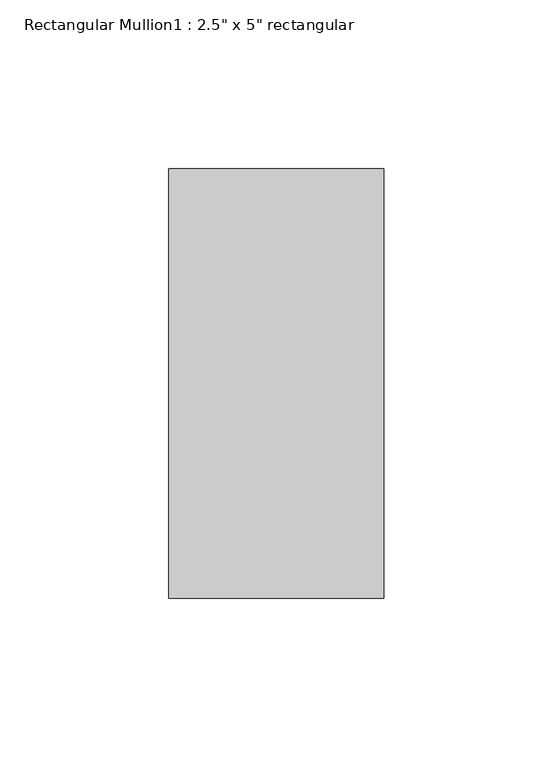
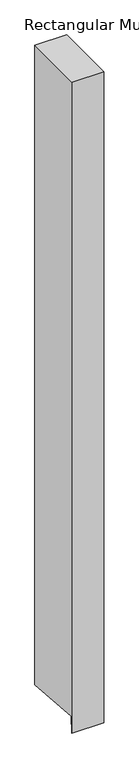
"""IFC4 building model written with IfcOpenShell, lengths in millimetres: member geometry."""

import ifcopenshell
import ifcopenshell.guid

model = None  # the IFC model being written
_history = None  # IfcOwnerHistory: only IFC2X3 demands one
_inside = {}  # id of a spatial element -> (the spatial element, [elements in it])
_under = {}  # id of a project, library or spatial element -> (it, [spatial elements below it])
_declared = {}  # id of a project -> (the project, [libraries it declares])
_typed = {}  # id of a type object -> (the type object, [elements of that type])
_made_of = {}  # id of a material, layer set ... -> (it, [elements and type objects made of it])


def new_model(schema):
    """Start an empty IFC model of exactly this schema.

    Asked for "IFC4X3", IfcOpenShell would pick the latest addendum, in which some entities
    have other attributes; the version numbers below select the first issue.
    IFC2X3 requires an IfcOwnerHistory on every rooted entity: one is made here for all.
    """
    global model, _history
    if schema == "IFC4X3":
        model = ifcopenshell.file(schema_version=(4, 3, 0, 0))
    else:
        model = ifcopenshell.file(schema=schema)
    _inside.clear()
    _under.clear()
    _declared.clear()
    _typed.clear()
    _made_of.clear()
    _history = None
    if model.schema == "IFC2X3":
        org = make("IfcOrganization", Name="unknown")
        user = make(
            "IfcPersonAndOrganization",
            ThePerson=make("IfcPerson", FamilyName="unknown"),
            TheOrganization=org,
        )
        app = make(
            "IfcApplication",
            ApplicationDeveloper=org,
            Version="unknown",
            ApplicationFullName="unknown",
            ApplicationIdentifier="unknown",
        )
        _history = make(
            "IfcOwnerHistory",
            OwningUser=user,
            OwningApplication=app,
            ChangeAction="ADDED",
            CreationDate=0,
        )
    return model


def make(cls, **values):
    """One entity of the class cls with the attributes given. An attribute that is None is left unset."""
    return model.create_entity(
        cls, **{name: value for name, value in values.items() if value is not None}
    )


def rooted(cls, **values):
    """An entity with a GlobalId (a new one), such as an element, a storey or a relation."""
    return make(cls, GlobalId=ifcopenshell.guid.new(), OwnerHistory=_history, **values)


def si_unit(unit_type, name, prefix=None):
    """IfcSIUnit, for example si_unit("LENGTHUNIT", "METRE", prefix="MILLI")."""
    return make("IfcSIUnit", UnitType=unit_type, Prefix=prefix, Name=name)


def assignment(units):
    """IfcUnitAssignment: the units of a project."""
    return None if units is None else make("IfcUnitAssignment", Units=units)


def point(xyz):
    """IfcCartesianPoint."""
    return None if xyz is None else make("IfcCartesianPoint", Coordinates=xyz)


def direction(xyz):
    """IfcDirection."""
    return None if xyz is None else make("IfcDirection", DirectionRatios=xyz)


def frame(location, z_axis=None, x_axis=None):
    """IfcAxis2Placement3D, a coordinate frame: its origin and axes. An axis left out is left unset."""
    return make(
        "IfcAxis2Placement3D",
        Location=point(location),
        Axis=direction(z_axis),
        RefDirection=direction(x_axis),
    )


def origin():
    """The frame at (0, 0, 0) with its axes left unset."""
    return frame((0.0, 0.0, 0.0))


def place(relative_to, where):
    """IfcLocalPlacement: puts the frame where relative to a parent placement (None: the world)."""
    return make(
        "IfcLocalPlacement", PlacementRelTo=relative_to, RelativePlacement=where
    )


def context(
    kind, dimensions, precision=None, world=None, true_north=None, identifier=None
):
    """IfcGeometricRepresentationContext, for example the 3D "Model" context."""
    return make(
        "IfcGeometricRepresentationContext",
        ContextIdentifier=identifier,
        ContextType=kind,
        CoordinateSpaceDimension=dimensions,
        Precision=precision,
        WorldCoordinateSystem=world,
        TrueNorth=true_north,
    )


def project(units=None, contexts=None):
    """IfcProject with its units and contexts."""
    return rooted(
        "IfcProject",
        Name="project",
        RepresentationContexts=contexts,
        UnitsInContext=assignment(units),
    )


def spatial(cls, under=None, at=None, **own):
    """A site, building, storey or space (cls), placed at a placement, below another one or the project."""
    s = rooted(cls, ObjectPlacement=at, **own)
    if under is not None:
        _under.setdefault(under.id(), (under, []))[1].append(s)
    return s


def polyline(points):
    """IfcPolyline through the points."""
    return make("IfcPolyline", Points=[point(p) for p in points])


def outline(outer, holes=None, kind="AREA"):
    """IfcArbitraryClosedProfileDef: a profile drawn as a closed curve; with holes, ...WithVoids."""
    if holes is None:
        return make("IfcArbitraryClosedProfileDef", ProfileType=kind, OuterCurve=outer)
    return make(
        "IfcArbitraryProfileDefWithVoids",
        ProfileType=kind,
        OuterCurve=outer,
        InnerCurves=holes,
    )


def extrude(swept, where, along, depth):
    """IfcExtrudedAreaSolid: the profile swept, set in the frame where, extruded along a direction by depth."""
    return make(
        "IfcExtrudedAreaSolid",
        SweptArea=swept,
        Position=where,
        ExtrudedDirection=direction(along),
        Depth=depth,
    )


def shape(context_of_items, identifier, shape_type, items):
    """IfcShapeRepresentation: the items that make up one representation, for example the "Body"."""
    return make(
        "IfcShapeRepresentation",
        ContextOfItems=context_of_items,
        RepresentationIdentifier=identifier,
        RepresentationType=shape_type,
        Items=items,
    )


def source(mapping_origin, context_of_items, identifier, shape_type, items):
    """IfcRepresentationMap: a shape defined once, which mapped items show again and again."""
    return make(
        "IfcRepresentationMap",
        MappingOrigin=mapping_origin,
        MappedRepresentation=shape(context_of_items, identifier, shape_type, items),
    )


def transform(
    local_origin,
    x_axis=None,
    y_axis=None,
    z_axis=None,
    scale=None,
    scale2=None,
    scale3=None,
    uniform=True,
):
    """IfcCartesianTransformationOperator3D, or its non-uniform kind. x_axis, y_axis, z_axis: its Axis1, 2, 3."""
    if uniform:
        return make(
            "IfcCartesianTransformationOperator3D",
            Axis1=direction(x_axis),
            Axis2=direction(y_axis),
            LocalOrigin=point(local_origin),
            Scale=scale,
            Axis3=direction(z_axis),
        )
    return make(
        "IfcCartesianTransformationOperator3DnonUniform",
        Axis1=direction(x_axis),
        Axis2=direction(y_axis),
        LocalOrigin=point(local_origin),
        Scale=scale,
        Axis3=direction(z_axis),
        Scale2=scale2,
        Scale3=scale3,
    )


def mapped(mapping_source, mapping_target):
    """IfcMappedItem: shows the shape of a source again, moved by a transform."""
    return make(
        "IfcMappedItem", MappingSource=mapping_source, MappingTarget=mapping_target
    )


def made_of(thing, what):
    """Note that an element or type object is made of a material, layer set ...; save() writes the relation."""
    if what is not None:
        _made_of.setdefault(what.id(), (what, []))[1].append(thing)
    return thing


def element(
    cls,
    number,
    at=None,
    inside=None,
    cuts=None,
    type_object=None,
    material=None,
    context=None,
    identifier="Body",
    shape_type=None,
    held_by="IfcProductDefinitionShape",
    body=None,
    shapes=None,
    **own,
):
    """One element of the class cls, such as IfcWall. Its Tag is "e" and its number.

    at: its placement. inside: the storey or other place that contains it. cuts: it is an
    opening in that element (IfcRelVoidsElement). A single representation is given by context,
    identifier, shape_type and body (its items); several are given by shapes. held_by: the class
    of the entity that holds the representations. save() writes the other relations.
    """
    e = rooted(cls, Tag="e%d" % number, ObjectPlacement=at, **own)
    if body is not None:
        shapes = [shape(context, identifier, shape_type, body)]
    if shapes is not None:
        e.Representation = make(held_by, Representations=shapes)
    if inside is not None:
        _inside.setdefault(inside.id(), (inside, []))[1].append(e)
    if cuts is not None:
        rooted(
            "IfcRelVoidsElement", RelatingBuildingElement=cuts, RelatedOpeningElement=e
        )
    if type_object is not None:
        _typed.setdefault(type_object.id(), (type_object, []))[1].append(e)
    return made_of(e, material)


def aggregate(whole, parts):
    """IfcRelAggregates: a whole, such as a stair, and the parts it consists of."""
    return rooted("IfcRelAggregates", RelatingObject=whole, RelatedObjects=parts)


def save(model, path):
    """Write the relations noted so far, then the file.

    IfcRelAggregates (storeys below a building ...), IfcRelContainedInSpatialStructure (elements
    in a storey), IfcRelDefinesByType, IfcRelAssociatesMaterial and IfcRelDeclares: one each for
    every whole, place, type object, material and project.
    """
    for whole, parts in _under.values():
        aggregate(whole, parts)
    for where, things in _inside.values():
        rooted(
            "IfcRelContainedInSpatialStructure",
            RelatedElements=things,
            RelatingStructure=where,
        )
    for kind, things in _typed.values():
        rooted("IfcRelDefinesByType", RelatedObjects=things, RelatingType=kind)
    for what, things in _made_of.values():
        rooted("IfcRelAssociatesMaterial", RelatedObjects=things, RelatingMaterial=what)
    for by, libraries in _declared.values():
        rooted("IfcRelDeclares", RelatingContext=by, RelatedDefinitions=libraries)
    model.write(path)


def member_2f5ef470(model_context):
    return source(origin(), model_context, "Body", "SweptSolid", [
        extrude(outline(polyline([(-63.5, 0.0), (63.5, 0.0), (63.5, -1344.0500431), (-60.9736199, -1334.8041085), (-63.5, -1368.815562), (-63.5, 0.0)])), frame((-63.5, 0.0, 0.0), z_axis=(1.0, 0.0, 0.0), x_axis=(0.0, 1.0, 0.0)), (0.0, 0.0, 1.0), 63.5),
    ])


if __name__ == "__main__":
    model = new_model("IFC4")
    model_context = context("Model", 3, world=origin())
    ifc_project = project(units=[si_unit("LENGTHUNIT", "METRE", prefix="MILLI")], contexts=[model_context])
    site = spatial("IfcSite", under=ifc_project)
    building = spatial("IfcBuilding", under=site)
    placement = place(None, origin())
    member_shape = member_2f5ef470(model_context)
    element("IfcMember", 1, ObjectType="Rectangular Mullion1 : 2.5\" x 5\" rectangular", at=placement, inside=building, context=model_context, shape_type="MappedRepresentation", body=[
        mapped(member_shape, transform((0.0, 0.0, 0.0), x_axis=(1.0, 0.0, 0.0), y_axis=(0.0, 1.0, 0.0), z_axis=(0.0, 0.0, 1.0))),
    ])
    save(model, "model.ifc")

# Revit data of these elements
# Type "Rectangular Mullion1 : 2.5\" x 5\" rectangular"
#   built-in parameter 1007304 = 0.416667 (stored number, unit not read)
#   built-in parameter 1007301 = 0.104167 (stored number, unit not read)
#   built-in parameter 1007300 = 0.104167 (stored number, unit not read)
# Element 1 (IfcMember, "Rectangular Mullion1 : 2.5\" x 5\" rectangular")
#   Materials on its faces: "support-frame"
# Materials
#   "support-frame": class "Unassigned", colour RGB 233 233 233, transparency 0, Cost = 0
